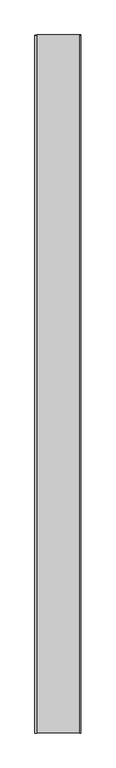
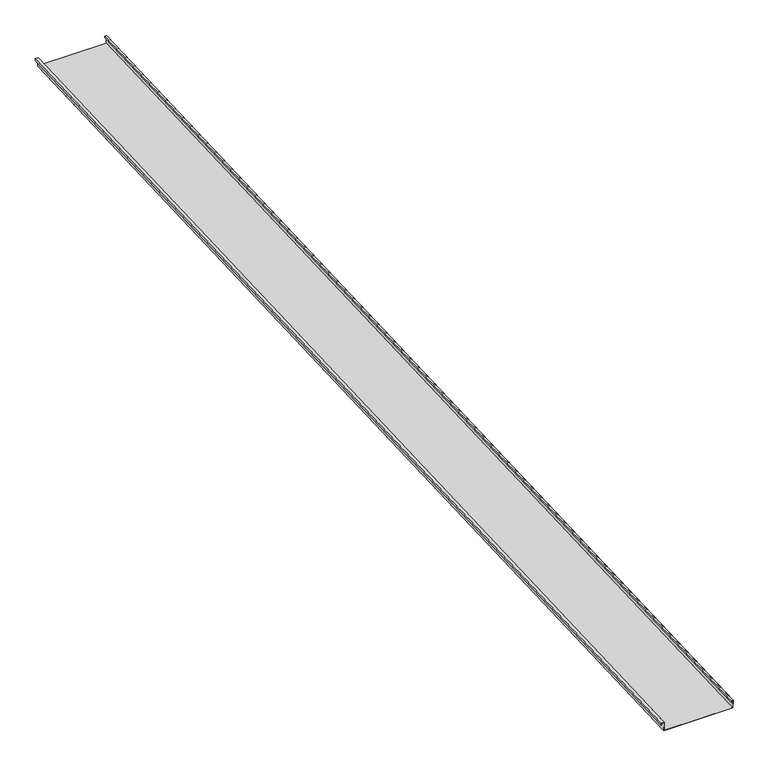
"""IFC4 building model written with IfcOpenShell, lengths in millimetres: proxy geometry, Generic Models 2:Generic Models 2:310765:Generic Models 2:310765 : Generic Models 2:Generic Models 2:310765:130 : Generic Models 2:Generic Models 2:310765:Generic Models 2:310765 : Generic Models 2:Generic Models 2:310765:300385."""

from ifc_helpers import new_model, si_unit, frame, origin, place, context, project, spatial, polyline, outline, extrude, source, transform, mapped, element, save


def generic_models_40906227(model_context):
    return source(origin(), model_context, "Body", "SweptSolid", [
        extrude(outline(polyline([(1.5875, 0.0), (1.5875, 50.8), (407.9875, 50.8), (407.9875, 1.5875), (396.875, 1.5875), (396.875, 11.1125), (398.4625, 11.1125), (398.4625, 3.175), (406.4, 3.175), (406.4, 49.2125), (3.175, 49.2125), (3.175, -1.5874999), (-14.2875, -1.5874999), (-14.2875, 9.525), (-12.7, 9.525), (-12.7, 0.0), (1.5875, 0.0)])), frame((660532.9429738, -581354.4345603, 3902.6697972), z_axis=(0.0, 0.9991330730923568, 0.041630544712067834), x_axis=(1.0, 0.0, 0.0)), (0.0, 0.0, 1.0), 6400.8),
    ])


if __name__ == "__main__":
    model = new_model("IFC4")
    model_context = context("Model", 3, world=origin())
    ifc_project = project(units=[si_unit("LENGTHUNIT", "METRE", prefix="MILLI")], contexts=[model_context])
    site = spatial("IfcSite", under=ifc_project)
    building = spatial("IfcBuilding", under=site)
    placement = place(None, origin())
    generic_models_shape = generic_models_40906227(model_context)
    element("IfcBuildingElementProxy", 1, Name="Generic Models 2:Generic Models 2:310765:Generic Models 2:310765 : Generic Models 2:Generic Models 2:310765:130 : Generic Models 2:Generic Models 2:310765:Generic Models 2:310765 : Generic Models 2:Generic Models 2:310765:300385", ObjectType="Generic Models 2:Generic Models 2:310765:Generic Models 2:310765 : Generic Models 2:Generic Models 2:310765:130 : Generic Models 2:Generic Models 2:310765:Generic Models 2:310765 : Generic Models 2:Generic Models 2:310765:300385", at=placement, inside=building, context=model_context, shape_type="MappedRepresentation", body=[
        mapped(generic_models_shape, transform((0.0, 0.0, 0.0), x_axis=(1.0, 0.0, 0.0), y_axis=(0.0, 1.0, 0.0), z_axis=(0.0, 0.0, 1.0))),
    ])
    save(model, "model.ifc")

# Revit data of these elements
# Type "Generic Models 2:Generic Models 2:310765:Generic Models 2:310765 : Generic Models 2:Generic Models 2:310765:130 : Generic Models 2:Generic Models 2:310765:Generic Models 2:310765 : Generic Models 2:Generic Models 2:310765:300385"
#   NameOverride = "Generic Models 2:Generic Models 2:310765:Generic Models 2:310765 : Generic Models 2:Generic Models 2:310765:300385"
#   ObjectTypeOverride = "Generic Models 2:310765 : Generic Models 2:Generic Models 2:310765"
#   Reference = "Generic Models 2"
#   Tag = "300385"
# Element 1 (IfcBuildingElementProxy, "Generic Models 2:Generic Models 2:310765:Generic Models 2:310765 : Generic Models 2:Generic Models 2:310765:130 : Generic Models 2:Generic Models 2:310765:Generic Models 2:310765 : Generic Models 2:Generic Models 2:310765:300385")
#   Materials on its faces: "THERMAL BROKEN ALUMINUM STOREFRONT FOR POLYCARBONATE"
# Materials
#   "THERMAL BROKEN ALUMINUM STOREFRONT FOR POLYCARBONATE": class "Unassigned", colour RGB 244 244 244, transparency 0, Keynote = "M07611300.01", Cost = 0
